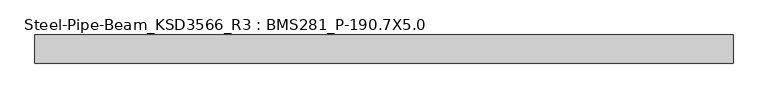
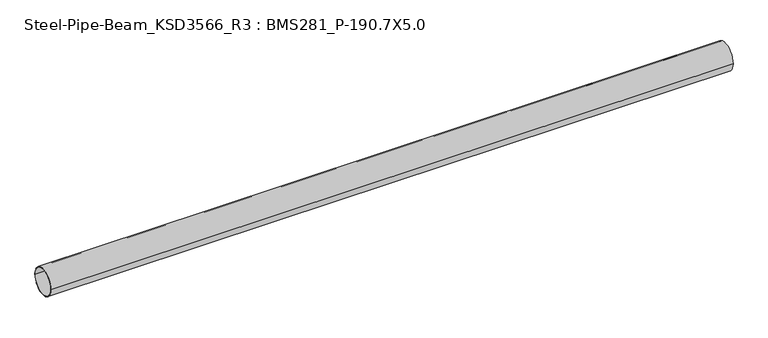
"""IFC4 building model written with IfcOpenShell, lengths in millimetres: member geometry, Steel-Pipe-Beam_KSD3566_R3 : BMS281_P-190.7X5.0."""

from ifc_helpers import new_model, si_unit, point, frame, origin, origin_2d, place, context, project, spatial, circle_curve, trimmed, segment, composite_curve, outline, extrude, source, transform, mapped, element, save


def steel_pipe_beam_ksd3566_r3_bms281_p_190_7x5_0_5e67390f(model_context):
    return source(origin(), model_context, "Body", "SweptSolid", [
        extrude(outline(composite_curve([segment(trimmed(circle_curve(origin_2d(), 95.35), [point((-95.35, 0.0))], [point((95.35, 0.0))], False, "CARTESIAN"), True, "CONTINUOUS"), segment(trimmed(circle_curve(origin_2d(), 95.35), [point((95.35, 0.0))], [point((-95.35, 0.0))], False, "CARTESIAN"), True, "CONTINUOUS")], self_intersect=False), holes=[composite_curve([segment(trimmed(circle_curve(origin_2d(), 90.35), [point((90.35, 0.0))], [point((-90.35, 0.0))], True, "CARTESIAN"), True, "CONTINUOUS"), segment(trimmed(circle_curve(origin_2d(), 90.35), [point((-90.35, 0.0))], [point((90.35, 0.0))], True, "CARTESIAN"), True, "CONTINUOUS")], self_intersect=False)]), frame((-2413.1370429, 0.0, 0.0), z_axis=(1.0, 0.0, 0.0), x_axis=(0.0, 1.0, 0.0)), (0.0, 0.0, 1.0), 4728.1627767),
    ])


if __name__ == "__main__":
    model = new_model("IFC4")
    model_context = context("Model", 3, world=origin())
    ifc_project = project(units=[si_unit("LENGTHUNIT", "METRE", prefix="MILLI")], contexts=[model_context])
    site = spatial("IfcSite", under=ifc_project)
    building = spatial("IfcBuilding", under=site)
    placement = place(None, origin())
    steel_pipe_beam_ksd3566_r3_bms281_p_190_7x5_0_shape = steel_pipe_beam_ksd3566_r3_bms281_p_190_7x5_0_5e67390f(model_context)
    element("IfcMember", 1, ObjectType="Steel-Pipe-Beam_KSD3566_R3 : BMS281_P-190.7X5.0", at=placement, inside=building, context=model_context, shape_type="MappedRepresentation", body=[
        mapped(steel_pipe_beam_ksd3566_r3_bms281_p_190_7x5_0_shape, transform((0.0, 0.0, 0.0), x_axis=(1.0, 0.0, 0.0), y_axis=(0.0, 1.0, 0.0), z_axis=(0.0, 0.0, 1.0))),
    ])
    save(model, "model.ifc")

# Revit data of these elements
# Type "Steel-Pipe-Beam_KSD3566_R3 : BMS281_P-190.7X5.0"
#   Keynote = "P-190.7X5.0"
#   SteelWeight = "Light"
#   t = 0.0050 m
#   Surface Area = 0.599102 m²/m
#   Section Area = 29.1697 cm²
#   Mass per Unit Length = 22.8982 kg/m
#   Length [instance default] = 1.5000 m
#   D = 0.1907 m
#   hec_material4 [instance default] = none
#   hec_material3 [instance default] = none
#   hec_material2 [instance default] = none
#   hec_material1 [instance default] = none
#   Structural Material [instance default] = Steel, 45-345
#   Assembly Code = ""
# Element 1 (IfcMember, "Steel-Pipe-Beam_KSD3566_R3 : BMS281_P-190.7X5.0")
#   Structural Material = none
# Materials
#   "Steel, 45-345": class "Metal", colour RGB 189 187 185, transparency 0, Description = "Steel 345 MPa", Cost = 0
